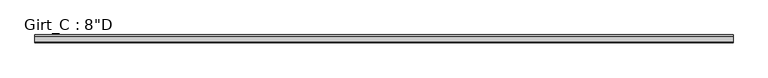
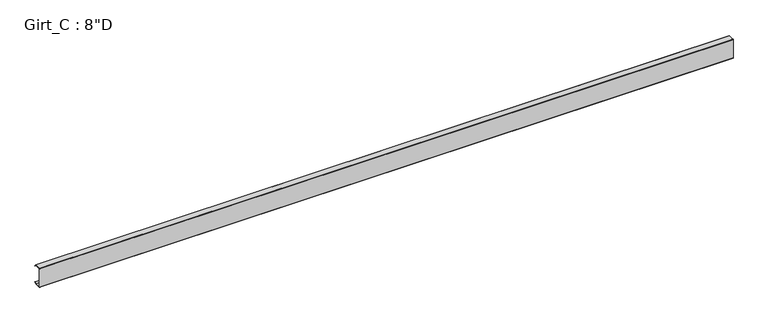
"""IFC4 building model written with IfcOpenShell, lengths in millimetres: beam geometry."""

from ifc_helpers import new_model, si_unit, point, frame, frame_2d, origin, place, context, project, spatial, polyline, circle_curve, trimmed, segment, composite_curve, outline, extrude, source, transform, mapped, element, save


def beam_ec662450(model_context):
    return source(origin(), model_context, "Body", "SweptSolid", [
        extrude(outline(composite_curve([segment(polyline([(63.5, 101.6), (75.745104, 87.0068534), (73.6169367, 85.221109), (62.204539, 98.821875), (3.3005807, 98.821875)]), True, "CONTINUOUS"), segment(trimmed(circle_curve(frame_2d((3.3741066, 96.8381931)), 1.9850441), [point((3.3005807, 98.821875))], [point((1.3890625, 96.8381931))], True, "CARTESIAN"), True, "CONTINUOUS"), segment(polyline([(1.3890625, 96.8381931), (1.3890625, -96.8389339)]), True, "CONTINUOUS"), segment(trimmed(circle_curve(frame_2d((3.3748024, -96.8389339)), 1.9857399), [point((1.3890625, -96.8389339))], [point((3.2694106, -98.821875))], True, "CARTESIAN"), True, "CONTINUOUS"), segment(polyline([(3.2694106, -98.821875), (62.204539, -98.821875), (73.6169367, -85.221109), (75.745104, -87.0068534), (63.5, -101.6), (3.3734375, -101.6)]), True, "CONTINUOUS"), segment(trimmed(circle_curve(frame_2d((3.3734375, -96.8375)), 4.7625), [point((3.3734375, -101.6))], [point((-1.3890625, -96.8375))], False, "CARTESIAN"), True, "CONTINUOUS"), segment(polyline([(-1.3890625, -96.8375), (-1.3890625, 96.8375)]), True, "CONTINUOUS"), segment(trimmed(circle_curve(frame_2d((3.3734375, 96.8375)), 4.7625), [point((-1.3890625, 96.8375))], [point((3.3734375, 101.6))], False, "CARTESIAN"), True, "CONTINUOUS"), segment(polyline([(3.3734375, 101.6), (63.5, 101.6)]), True, "CONTINUOUS")], self_intersect=False)), frame((-3566.31875, 0.0, 0.0), z_axis=(1.0, 0.0, 0.0), x_axis=(0.0, 1.0, 0.0)), (0.0, 0.0, 1.0), 6972.3),
    ])


if __name__ == "__main__":
    model = new_model("IFC4")
    model_context = context("Model", 3, world=origin())
    ifc_project = project(units=[si_unit("LENGTHUNIT", "METRE", prefix="MILLI")], contexts=[model_context])
    site = spatial("IfcSite", under=ifc_project)
    building = spatial("IfcBuilding", under=site)
    placement = place(None, origin())
    beam_shape = beam_ec662450(model_context)
    element("IfcBeam", 1, ObjectType="Girt_C : 8\"D", at=placement, inside=building, context=model_context, shape_type="MappedRepresentation", body=[
        mapped(beam_shape, transform((0.0, 0.0, 0.0), x_axis=(1.0, 0.0, 0.0), y_axis=(0.0, 1.0, 0.0), z_axis=(0.0, 0.0, 1.0))),
    ])
    save(model, "model.ifc")

# Revit data of these elements
# Type "Girt_C : 8\"D"
#   Web_Thickness = 0' - 0 7/64"
#   Length [instance default] = 10' - 0"
#   Leg_1 = 0' - 2 1/2"
#   Height = 0' - 8"
#   Structural Material [instance default] = none
# Element 1 (IfcBeam, "Girt_C : 8\"D")
#   Structural Material = Steel
#   Materials on its faces: "Steel"
# Materials
#   "Steel": class "Metal", colour RGB 118 118 114, transparency 0, Description = "Steel, mill finish", Cost = 0
